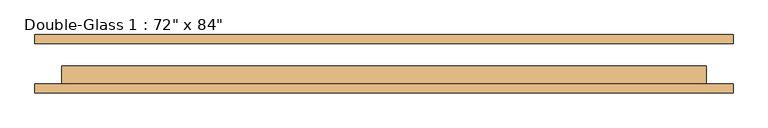
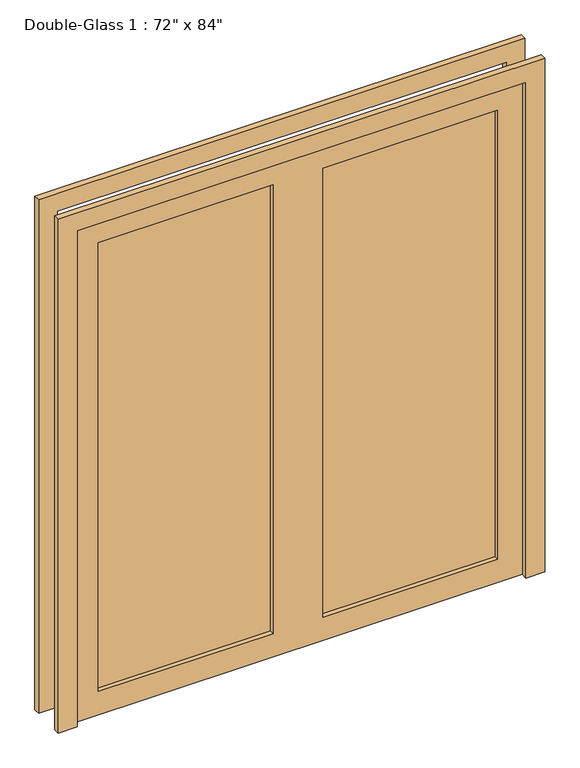
"""IFC4 building model written with IfcOpenShell, lengths in millimetres: door geometry."""

import ifcopenshell
import ifcopenshell.guid

model = None  # the IFC model being written
_history = None  # IfcOwnerHistory: only IFC2X3 demands one
_inside = {}  # id of a spatial element -> (the spatial element, [elements in it])
_under = {}  # id of a project, library or spatial element -> (it, [spatial elements below it])
_declared = {}  # id of a project -> (the project, [libraries it declares])
_typed = {}  # id of a type object -> (the type object, [elements of that type])
_made_of = {}  # id of a material, layer set ... -> (it, [elements and type objects made of it])


def new_model(schema):
    """Start an empty IFC model of exactly this schema.

    Asked for "IFC4X3", IfcOpenShell would pick the latest addendum, in which some entities
    have other attributes; the version numbers below select the first issue.
    IFC2X3 requires an IfcOwnerHistory on every rooted entity: one is made here for all.
    """
    global model, _history
    if schema == "IFC4X3":
        model = ifcopenshell.file(schema_version=(4, 3, 0, 0))
    else:
        model = ifcopenshell.file(schema=schema)
    _inside.clear()
    _under.clear()
    _declared.clear()
    _typed.clear()
    _made_of.clear()
    _history = None
    if model.schema == "IFC2X3":
        org = make("IfcOrganization", Name="unknown")
        user = make(
            "IfcPersonAndOrganization",
            ThePerson=make("IfcPerson", FamilyName="unknown"),
            TheOrganization=org,
        )
        app = make(
            "IfcApplication",
            ApplicationDeveloper=org,
            Version="unknown",
            ApplicationFullName="unknown",
            ApplicationIdentifier="unknown",
        )
        _history = make(
            "IfcOwnerHistory",
            OwningUser=user,
            OwningApplication=app,
            ChangeAction="ADDED",
            CreationDate=0,
        )
    return model


def make(cls, **values):
    """One entity of the class cls with the attributes given. An attribute that is None is left unset."""
    return model.create_entity(
        cls, **{name: value for name, value in values.items() if value is not None}
    )


def rooted(cls, **values):
    """An entity with a GlobalId (a new one), such as an element, a storey or a relation."""
    return make(cls, GlobalId=ifcopenshell.guid.new(), OwnerHistory=_history, **values)


def si_unit(unit_type, name, prefix=None):
    """IfcSIUnit, for example si_unit("LENGTHUNIT", "METRE", prefix="MILLI")."""
    return make("IfcSIUnit", UnitType=unit_type, Prefix=prefix, Name=name)


def assignment(units):
    """IfcUnitAssignment: the units of a project."""
    return None if units is None else make("IfcUnitAssignment", Units=units)


def point(xyz):
    """IfcCartesianPoint."""
    return None if xyz is None else make("IfcCartesianPoint", Coordinates=xyz)


def direction(xyz):
    """IfcDirection."""
    return None if xyz is None else make("IfcDirection", DirectionRatios=xyz)


def frame(location, z_axis=None, x_axis=None):
    """IfcAxis2Placement3D, a coordinate frame: its origin and axes. An axis left out is left unset."""
    return make(
        "IfcAxis2Placement3D",
        Location=point(location),
        Axis=direction(z_axis),
        RefDirection=direction(x_axis),
    )


def origin():
    """The frame at (0, 0, 0) with its axes left unset."""
    return frame((0.0, 0.0, 0.0))


def place(relative_to, where):
    """IfcLocalPlacement: puts the frame where relative to a parent placement (None: the world)."""
    return make(
        "IfcLocalPlacement", PlacementRelTo=relative_to, RelativePlacement=where
    )


def context(
    kind, dimensions, precision=None, world=None, true_north=None, identifier=None
):
    """IfcGeometricRepresentationContext, for example the 3D "Model" context."""
    return make(
        "IfcGeometricRepresentationContext",
        ContextIdentifier=identifier,
        ContextType=kind,
        CoordinateSpaceDimension=dimensions,
        Precision=precision,
        WorldCoordinateSystem=world,
        TrueNorth=true_north,
    )


def project(units=None, contexts=None):
    """IfcProject with its units and contexts."""
    return rooted(
        "IfcProject",
        Name="project",
        RepresentationContexts=contexts,
        UnitsInContext=assignment(units),
    )


def spatial(cls, under=None, at=None, **own):
    """A site, building, storey or space (cls), placed at a placement, below another one or the project."""
    s = rooted(cls, ObjectPlacement=at, **own)
    if under is not None:
        _under.setdefault(under.id(), (under, []))[1].append(s)
    return s


def polyline(points):
    """IfcPolyline through the points."""
    return make("IfcPolyline", Points=[point(p) for p in points])


def outline(outer, holes=None, kind="AREA"):
    """IfcArbitraryClosedProfileDef: a profile drawn as a closed curve; with holes, ...WithVoids."""
    if holes is None:
        return make("IfcArbitraryClosedProfileDef", ProfileType=kind, OuterCurve=outer)
    return make(
        "IfcArbitraryProfileDefWithVoids",
        ProfileType=kind,
        OuterCurve=outer,
        InnerCurves=holes,
    )


def extrude(swept, where, along, depth):
    """IfcExtrudedAreaSolid: the profile swept, set in the frame where, extruded along a direction by depth."""
    return make(
        "IfcExtrudedAreaSolid",
        SweptArea=swept,
        Position=where,
        ExtrudedDirection=direction(along),
        Depth=depth,
    )


def shape(context_of_items, identifier, shape_type, items):
    """IfcShapeRepresentation: the items that make up one representation, for example the "Body"."""
    return make(
        "IfcShapeRepresentation",
        ContextOfItems=context_of_items,
        RepresentationIdentifier=identifier,
        RepresentationType=shape_type,
        Items=items,
    )


def source(mapping_origin, context_of_items, identifier, shape_type, items):
    """IfcRepresentationMap: a shape defined once, which mapped items show again and again."""
    return make(
        "IfcRepresentationMap",
        MappingOrigin=mapping_origin,
        MappedRepresentation=shape(context_of_items, identifier, shape_type, items),
    )


def transform(
    local_origin,
    x_axis=None,
    y_axis=None,
    z_axis=None,
    scale=None,
    scale2=None,
    scale3=None,
    uniform=True,
):
    """IfcCartesianTransformationOperator3D, or its non-uniform kind. x_axis, y_axis, z_axis: its Axis1, 2, 3."""
    if uniform:
        return make(
            "IfcCartesianTransformationOperator3D",
            Axis1=direction(x_axis),
            Axis2=direction(y_axis),
            LocalOrigin=point(local_origin),
            Scale=scale,
            Axis3=direction(z_axis),
        )
    return make(
        "IfcCartesianTransformationOperator3DnonUniform",
        Axis1=direction(x_axis),
        Axis2=direction(y_axis),
        LocalOrigin=point(local_origin),
        Scale=scale,
        Axis3=direction(z_axis),
        Scale2=scale2,
        Scale3=scale3,
    )


def mapped(mapping_source, mapping_target):
    """IfcMappedItem: shows the shape of a source again, moved by a transform."""
    return make(
        "IfcMappedItem", MappingSource=mapping_source, MappingTarget=mapping_target
    )


def made_of(thing, what):
    """Note that an element or type object is made of a material, layer set ...; save() writes the relation."""
    if what is not None:
        _made_of.setdefault(what.id(), (what, []))[1].append(thing)
    return thing


def element(
    cls,
    number,
    at=None,
    inside=None,
    cuts=None,
    type_object=None,
    material=None,
    context=None,
    identifier="Body",
    shape_type=None,
    held_by="IfcProductDefinitionShape",
    body=None,
    shapes=None,
    **own,
):
    """One element of the class cls, such as IfcWall. Its Tag is "e" and its number.

    at: its placement. inside: the storey or other place that contains it. cuts: it is an
    opening in that element (IfcRelVoidsElement). A single representation is given by context,
    identifier, shape_type and body (its items); several are given by shapes. held_by: the class
    of the entity that holds the representations. save() writes the other relations.
    """
    e = rooted(cls, Tag="e%d" % number, ObjectPlacement=at, **own)
    if body is not None:
        shapes = [shape(context, identifier, shape_type, body)]
    if shapes is not None:
        e.Representation = make(held_by, Representations=shapes)
    if inside is not None:
        _inside.setdefault(inside.id(), (inside, []))[1].append(e)
    if cuts is not None:
        rooted(
            "IfcRelVoidsElement", RelatingBuildingElement=cuts, RelatedOpeningElement=e
        )
    if type_object is not None:
        _typed.setdefault(type_object.id(), (type_object, []))[1].append(e)
    return made_of(e, material)


def aggregate(whole, parts):
    """IfcRelAggregates: a whole, such as a stair, and the parts it consists of."""
    return rooted("IfcRelAggregates", RelatingObject=whole, RelatedObjects=parts)


def save(model, path):
    """Write the relations noted so far, then the file.

    IfcRelAggregates (storeys below a building ...), IfcRelContainedInSpatialStructure (elements
    in a storey), IfcRelDefinesByType, IfcRelAssociatesMaterial and IfcRelDeclares: one each for
    every whole, place, type object, material and project.
    """
    for whole, parts in _under.values():
        aggregate(whole, parts)
    for where, things in _inside.values():
        rooted(
            "IfcRelContainedInSpatialStructure",
            RelatedElements=things,
            RelatingStructure=where,
        )
    for kind, things in _typed.values():
        rooted("IfcRelDefinesByType", RelatedObjects=things, RelatingType=kind)
    for what, things in _made_of.values():
        rooted("IfcRelAssociatesMaterial", RelatedObjects=things, RelatingMaterial=what)
    for by, libraries in _declared.values():
        rooted("IfcRelDeclares", RelatingContext=by, RelatedDefinitions=libraries)
    model.write(path)


def door_6bc470f4(model_context):
    return source(origin(), model_context, "Body", "SweptSolid", [
        extrude(outline(polyline([(0.0, 990.6), (2209.8, 990.6), (2209.8, -990.6), (0.0, -990.6), (0.0, -914.4), (2133.6, -914.4), (2133.6, 914.4), (0.0, 914.4), (0.0, 990.6)])), frame((0.0, 54.76875, 0.0), z_axis=(0.0, 1.0, 0.0), x_axis=(0.0, 0.0, 1.0)), (0.0, 0.0, 1.0), 25.4),
        extrude(outline(polyline([(2133.6, 914.4), (0.0, 914.4), (0.0, 990.6), (2209.8, 990.6), (2209.8, -990.6), (0.0, -990.6), (0.0, -914.4), (2133.6, -914.4), (2133.6, 914.4)])), frame((0.0, -84.93125, 0.0), z_axis=(0.0, 1.0, 0.0), x_axis=(0.0, 0.0, 1.0)), (0.0, 0.0, 1.0), 25.4),
        extrude(outline(polyline([(812.8, -34.13125), (812.8, -41.275), (101.6, -41.275), (101.6, -34.13125), (812.8, -34.13125)])), frame((0.0, 0.0, 101.6), z_axis=(0.0, 0.0, 1.0), x_axis=(1.0, 0.0, 0.0)), (0.0, 0.0, 1.0), 1930.4),
        extrude(outline(polyline([(-101.6, -34.13125), (-101.6, -41.275), (-812.8, -41.275), (-812.8, -34.13125), (-101.6, -34.13125)])), frame((0.0, 0.0, 101.6), z_axis=(0.0, 0.0, 1.0), x_axis=(1.0, 0.0, 0.0)), (0.0, 0.0, 1.0), 1930.4),
        extrude(outline(polyline([(2133.6, 914.4), (2133.6, -914.4), (0.0, -914.4), (0.0, 914.4), (2133.6, 914.4)]), holes=[polyline([(2032.0, -101.6), (101.6, -101.6), (101.6, -812.8), (2032.0, -812.8), (2032.0, -101.6)]), polyline([(2032.0, 812.8), (101.6, 812.8), (101.6, 101.6), (2032.0, 101.6), (2032.0, 812.8)])]), frame((0.0, -59.53125, 0.0), z_axis=(0.0, 1.0, 0.0), x_axis=(0.0, 0.0, 1.0)), (0.0, 0.0, 1.0), 50.8),
    ])


if __name__ == "__main__":
    model = new_model("IFC4")
    model_context = context("Model", 3, world=origin())
    ifc_project = project(units=[si_unit("LENGTHUNIT", "METRE", prefix="MILLI")], contexts=[model_context])
    site = spatial("IfcSite", under=ifc_project)
    building = spatial("IfcBuilding", under=site)
    placement = place(None, origin())
    door_shape = door_6bc470f4(model_context)
    element("IfcDoor", 1, ObjectType="Double-Glass 1 : 72\" x 84\"", at=placement, inside=building, context=model_context, shape_type="MappedRepresentation", body=[
        mapped(door_shape, transform((0.0, 0.0, 0.0), x_axis=(1.0, 0.0, 0.0), y_axis=(0.0, 1.0, 0.0), z_axis=(0.0, 0.0, 1.0))),
    ])
    save(model, "model.ifc")

# Revit data of these elements
# Type "Double-Glass 1 : 72\" x 84\""
#   Type Mark = "34"
#   Assembly Code = "C1020"
#   Thickness = 0' - 2"
#   Height = 7' - 0"
#   Rail Width - Base = 0' - 4"
#   Rail Width - Top = 0' - 4"
#   Stile Width - Hinge = 0' - 4"
#   Stile Width - Latch = 0' - 4"
#   Trim Projection = 0' - 1"
#   Trim Width = 0' - 3"
#   Width = 6' - 0"
#   Function = 0
#   Door Material = Door - Panel
#   Frame Material = Door - Frame
#   Wall Closure = (empty or 0)
# Element 1 (IfcDoor, "Double-Glass 1 : 72\" x 84\"")
#   Materials on its faces: "Door - Frame", "Door - Panel", "Glass"
# Materials
#   "Door - Panel": class "Wood", colour RGB 230 193 158, transparency 0, Cost = 0
#   "Door - Frame": class "Paint", colour RGB 113 0 0, transparency 0, Cost = 0
#   "Glass": class "Glass", colour RGB 0 128 192, transparency 0.75, Cost = 0
